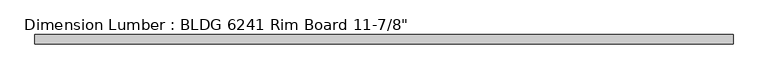
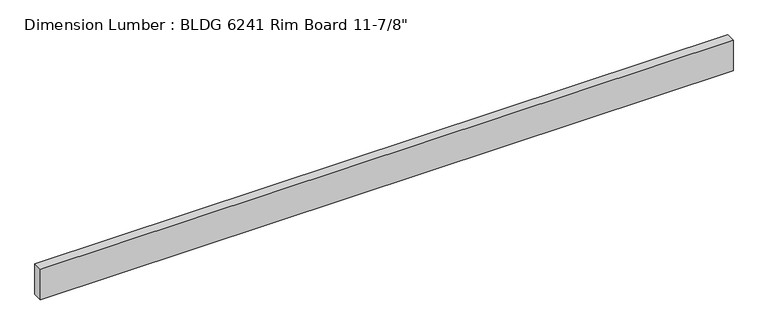
"""IFC4 building model written with IfcOpenShell, lengths in millimetres: beam geometry."""

import ifcopenshell
import ifcopenshell.guid

model = None  # the IFC model being written
_history = None  # IfcOwnerHistory: only IFC2X3 demands one
_inside = {}  # id of a spatial element -> (the spatial element, [elements in it])
_under = {}  # id of a project, library or spatial element -> (it, [spatial elements below it])
_declared = {}  # id of a project -> (the project, [libraries it declares])
_typed = {}  # id of a type object -> (the type object, [elements of that type])
_made_of = {}  # id of a material, layer set ... -> (it, [elements and type objects made of it])


def new_model(schema):
    """Start an empty IFC model of exactly this schema.

    Asked for "IFC4X3", IfcOpenShell would pick the latest addendum, in which some entities
    have other attributes; the version numbers below select the first issue.
    IFC2X3 requires an IfcOwnerHistory on every rooted entity: one is made here for all.
    """
    global model, _history
    if schema == "IFC4X3":
        model = ifcopenshell.file(schema_version=(4, 3, 0, 0))
    else:
        model = ifcopenshell.file(schema=schema)
    _inside.clear()
    _under.clear()
    _declared.clear()
    _typed.clear()
    _made_of.clear()
    _history = None
    if model.schema == "IFC2X3":
        org = make("IfcOrganization", Name="unknown")
        user = make(
            "IfcPersonAndOrganization",
            ThePerson=make("IfcPerson", FamilyName="unknown"),
            TheOrganization=org,
        )
        app = make(
            "IfcApplication",
            ApplicationDeveloper=org,
            Version="unknown",
            ApplicationFullName="unknown",
            ApplicationIdentifier="unknown",
        )
        _history = make(
            "IfcOwnerHistory",
            OwningUser=user,
            OwningApplication=app,
            ChangeAction="ADDED",
            CreationDate=0,
        )
    return model


def make(cls, **values):
    """One entity of the class cls with the attributes given. An attribute that is None is left unset."""
    return model.create_entity(
        cls, **{name: value for name, value in values.items() if value is not None}
    )


def rooted(cls, **values):
    """An entity with a GlobalId (a new one), such as an element, a storey or a relation."""
    return make(cls, GlobalId=ifcopenshell.guid.new(), OwnerHistory=_history, **values)


def si_unit(unit_type, name, prefix=None):
    """IfcSIUnit, for example si_unit("LENGTHUNIT", "METRE", prefix="MILLI")."""
    return make("IfcSIUnit", UnitType=unit_type, Prefix=prefix, Name=name)


def assignment(units):
    """IfcUnitAssignment: the units of a project."""
    return None if units is None else make("IfcUnitAssignment", Units=units)


def point(xyz):
    """IfcCartesianPoint."""
    return None if xyz is None else make("IfcCartesianPoint", Coordinates=xyz)


def direction(xyz):
    """IfcDirection."""
    return None if xyz is None else make("IfcDirection", DirectionRatios=xyz)


def frame(location, z_axis=None, x_axis=None):
    """IfcAxis2Placement3D, a coordinate frame: its origin and axes. An axis left out is left unset."""
    return make(
        "IfcAxis2Placement3D",
        Location=point(location),
        Axis=direction(z_axis),
        RefDirection=direction(x_axis),
    )


def origin():
    """The frame at (0, 0, 0) with its axes left unset."""
    return frame((0.0, 0.0, 0.0))


def place(relative_to, where):
    """IfcLocalPlacement: puts the frame where relative to a parent placement (None: the world)."""
    return make(
        "IfcLocalPlacement", PlacementRelTo=relative_to, RelativePlacement=where
    )


def context(
    kind, dimensions, precision=None, world=None, true_north=None, identifier=None
):
    """IfcGeometricRepresentationContext, for example the 3D "Model" context."""
    return make(
        "IfcGeometricRepresentationContext",
        ContextIdentifier=identifier,
        ContextType=kind,
        CoordinateSpaceDimension=dimensions,
        Precision=precision,
        WorldCoordinateSystem=world,
        TrueNorth=true_north,
    )


def project(units=None, contexts=None):
    """IfcProject with its units and contexts."""
    return rooted(
        "IfcProject",
        Name="project",
        RepresentationContexts=contexts,
        UnitsInContext=assignment(units),
    )


def spatial(cls, under=None, at=None, **own):
    """A site, building, storey or space (cls), placed at a placement, below another one or the project."""
    s = rooted(cls, ObjectPlacement=at, **own)
    if under is not None:
        _under.setdefault(under.id(), (under, []))[1].append(s)
    return s


def polyline(points):
    """IfcPolyline through the points."""
    return make("IfcPolyline", Points=[point(p) for p in points])


def outline(outer, holes=None, kind="AREA"):
    """IfcArbitraryClosedProfileDef: a profile drawn as a closed curve; with holes, ...WithVoids."""
    if holes is None:
        return make("IfcArbitraryClosedProfileDef", ProfileType=kind, OuterCurve=outer)
    return make(
        "IfcArbitraryProfileDefWithVoids",
        ProfileType=kind,
        OuterCurve=outer,
        InnerCurves=holes,
    )


def extrude(swept, where, along, depth):
    """IfcExtrudedAreaSolid: the profile swept, set in the frame where, extruded along a direction by depth."""
    return make(
        "IfcExtrudedAreaSolid",
        SweptArea=swept,
        Position=where,
        ExtrudedDirection=direction(along),
        Depth=depth,
    )


def shape(context_of_items, identifier, shape_type, items):
    """IfcShapeRepresentation: the items that make up one representation, for example the "Body"."""
    return make(
        "IfcShapeRepresentation",
        ContextOfItems=context_of_items,
        RepresentationIdentifier=identifier,
        RepresentationType=shape_type,
        Items=items,
    )


def source(mapping_origin, context_of_items, identifier, shape_type, items):
    """IfcRepresentationMap: a shape defined once, which mapped items show again and again."""
    return make(
        "IfcRepresentationMap",
        MappingOrigin=mapping_origin,
        MappedRepresentation=shape(context_of_items, identifier, shape_type, items),
    )


def transform(
    local_origin,
    x_axis=None,
    y_axis=None,
    z_axis=None,
    scale=None,
    scale2=None,
    scale3=None,
    uniform=True,
):
    """IfcCartesianTransformationOperator3D, or its non-uniform kind. x_axis, y_axis, z_axis: its Axis1, 2, 3."""
    if uniform:
        return make(
            "IfcCartesianTransformationOperator3D",
            Axis1=direction(x_axis),
            Axis2=direction(y_axis),
            LocalOrigin=point(local_origin),
            Scale=scale,
            Axis3=direction(z_axis),
        )
    return make(
        "IfcCartesianTransformationOperator3DnonUniform",
        Axis1=direction(x_axis),
        Axis2=direction(y_axis),
        LocalOrigin=point(local_origin),
        Scale=scale,
        Axis3=direction(z_axis),
        Scale2=scale2,
        Scale3=scale3,
    )


def mapped(mapping_source, mapping_target):
    """IfcMappedItem: shows the shape of a source again, moved by a transform."""
    return make(
        "IfcMappedItem", MappingSource=mapping_source, MappingTarget=mapping_target
    )


def made_of(thing, what):
    """Note that an element or type object is made of a material, layer set ...; save() writes the relation."""
    if what is not None:
        _made_of.setdefault(what.id(), (what, []))[1].append(thing)
    return thing


def element(
    cls,
    number,
    at=None,
    inside=None,
    cuts=None,
    type_object=None,
    material=None,
    context=None,
    identifier="Body",
    shape_type=None,
    held_by="IfcProductDefinitionShape",
    body=None,
    shapes=None,
    **own,
):
    """One element of the class cls, such as IfcWall. Its Tag is "e" and its number.

    at: its placement. inside: the storey or other place that contains it. cuts: it is an
    opening in that element (IfcRelVoidsElement). A single representation is given by context,
    identifier, shape_type and body (its items); several are given by shapes. held_by: the class
    of the entity that holds the representations. save() writes the other relations.
    """
    e = rooted(cls, Tag="e%d" % number, ObjectPlacement=at, **own)
    if body is not None:
        shapes = [shape(context, identifier, shape_type, body)]
    if shapes is not None:
        e.Representation = make(held_by, Representations=shapes)
    if inside is not None:
        _inside.setdefault(inside.id(), (inside, []))[1].append(e)
    if cuts is not None:
        rooted(
            "IfcRelVoidsElement", RelatingBuildingElement=cuts, RelatedOpeningElement=e
        )
    if type_object is not None:
        _typed.setdefault(type_object.id(), (type_object, []))[1].append(e)
    return made_of(e, material)


def aggregate(whole, parts):
    """IfcRelAggregates: a whole, such as a stair, and the parts it consists of."""
    return rooted("IfcRelAggregates", RelatingObject=whole, RelatedObjects=parts)


def save(model, path):
    """Write the relations noted so far, then the file.

    IfcRelAggregates (storeys below a building ...), IfcRelContainedInSpatialStructure (elements
    in a storey), IfcRelDefinesByType, IfcRelAssociatesMaterial and IfcRelDeclares: one each for
    every whole, place, type object, material and project.
    """
    for whole, parts in _under.values():
        aggregate(whole, parts)
    for where, things in _inside.values():
        rooted(
            "IfcRelContainedInSpatialStructure",
            RelatedElements=things,
            RelatingStructure=where,
        )
    for kind, things in _typed.values():
        rooted("IfcRelDefinesByType", RelatedObjects=things, RelatingType=kind)
    for what, things in _made_of.values():
        rooted("IfcRelAssociatesMaterial", RelatedObjects=things, RelatingMaterial=what)
    for by, libraries in _declared.values():
        rooted("IfcRelDeclares", RelatingContext=by, RelatedDefinitions=libraries)
    model.write(path)


def beam_440427b1(model_context):
    return source(origin(), model_context, "Body", "SweptSolid", [
        extrude(outline(polyline([(3254.375, 44.45), (3254.375, -44.45), (-3254.375, -44.45), (-3254.375, 44.45), (3254.375, 44.45)])), frame((0.0, 0.0, -150.8125), z_axis=(0.0, 0.0, 1.0), x_axis=(1.0, 0.0, 0.0)), (0.0, 0.0, 1.0), 301.625),
    ])


if __name__ == "__main__":
    model = new_model("IFC4")
    model_context = context("Model", 3, world=origin())
    ifc_project = project(units=[si_unit("LENGTHUNIT", "METRE", prefix="MILLI")], contexts=[model_context])
    site = spatial("IfcSite", under=ifc_project)
    building = spatial("IfcBuilding", under=site)
    placement = place(None, origin())
    beam_shape = beam_440427b1(model_context)
    element("IfcBeam", 1, ObjectType="Dimension Lumber : BLDG 6241 Rim Board 11-7/8\"", at=placement, inside=building, context=model_context, shape_type="MappedRepresentation", body=[
        mapped(beam_shape, transform((0.0, 0.0, 0.0), x_axis=(1.0, 0.0, 0.0), y_axis=(0.0, 1.0, 0.0), z_axis=(0.0, 0.0, 1.0))),
    ])
    save(model, "model.ifc")

# Revit data of these elements
# Type "Dimension Lumber : BLDG 6241 Rim Board 11-7/8\""
#   Assembly Code = "B10"
#   A = 0.273472 SF
#   Length [instance default] = 5' - 0"
#   b = 0' - 3 1/2"
#   d = 0' - 11 7/8"
#   Structural Material [instance default] = Softwood, Lumber
# Element 1 (IfcBeam, "Dimension Lumber : BLDG 6241 Rim Board 11-7/8\"")
#   Materials on its faces: "Softwood, Lumber"
# Materials
#   "Softwood, Lumber": class "Wood", colour RGB 223 192 134, transparency 0, Description = "Pinus Echinata", Cost = 0
